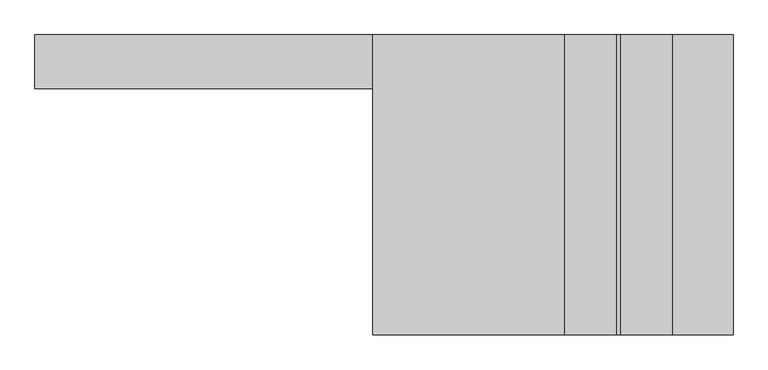
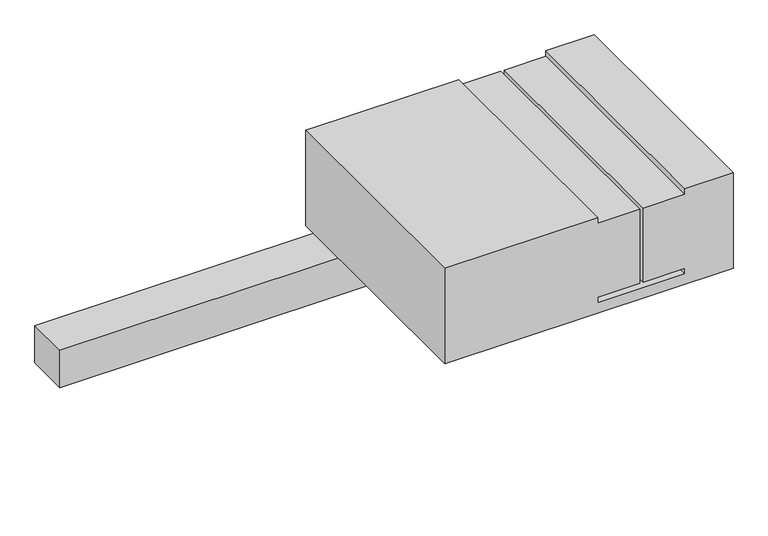
"""IFC4 building model written with IfcOpenShell, lengths in millimetres: proxy geometry, Framing058 14884 : Framing058 14884."""

from ifc_helpers import new_model, si_unit, frame, origin, place, context, project, spatial, polyline, outline, extrude, source, transform, mapped, element, save


def generic_models_ac43adbf(model_context):
    return source(origin(), model_context, "Body", "SweptSolid", [
        extrude(outline(polyline([(39757.096, -718.8864422), (40112.696, -718.8864422), (40112.696, -889.0664422), (40092.122, -889.0664422), (40092.122, -1036.1959422), (39815.77, -1036.1959422), (39815.77, -889.0664422), (39795.196, -889.0664422), (39795.196, -1196.4064422), (39815.77, -1196.4064422), (39815.77, -1049.2769422), (40092.122, -1049.2769422), (40092.122, -1196.4064422), (40112.696, -1196.4064422), (40112.696, -1738.0614422), (39757.096, -1738.0614422), (39757.096, -718.8864422)])), frame((0.0, 96.9874752, 0.0), z_axis=(0.0, 1.0, 0.0), x_axis=(0.0, 0.0, 1.0)), (0.0, 0.0, 1.0), 850.1218674),
        extrude(outline(polyline([(-718.8864422, 794.7093426), (-2694.3737014, 794.7093426), (-2694.3737014, 947.1093426), (-718.8864422, 947.1093426), (-718.8864422, 794.7093426)])), frame((0.0, 0.0, 39579.2960083), z_axis=(0.0, 0.0, 1.0), x_axis=(1.0, 0.0, 0.0)), (0.0, 0.0, 1.0), 139.7),
    ])


if __name__ == "__main__":
    model = new_model("IFC4")
    model_context = context("Model", 3, world=origin())
    ifc_project = project(units=[si_unit("LENGTHUNIT", "METRE", prefix="MILLI")], contexts=[model_context])
    site = spatial("IfcSite", under=ifc_project)
    building = spatial("IfcBuilding", under=site)
    placement = place(None, origin())
    generic_models_shape = generic_models_ac43adbf(model_context)
    element("IfcBuildingElementProxy", 1, Name="Framing058 14884 : Framing058 14884", ObjectType="Framing058 14884 : Framing058 14884", at=placement, inside=building, context=model_context, shape_type="MappedRepresentation", body=[
        mapped(generic_models_shape, transform((0.0, 0.0, 0.0), x_axis=(1.0, 0.0, 0.0), y_axis=(0.0, 1.0, 0.0), z_axis=(0.0, 0.0, 1.0))),
    ])
    save(model, "model.ifc")

# Revit data of these elements
# Type "Framing058 14884 : Framing058 14884"
#   NameOverride = "Framing058"
# Element 1 (IfcBuildingElementProxy, "Framing058 14884 : Framing058 14884")
#   Materials on its faces: "WOOD FRAMING (SEE STRUCT DWGS)"
# Materials
#   "WOOD FRAMING (SEE STRUCT DWGS)": class "Unassigned", colour RGB 224 188 168, transparency 0, Cost = 0
